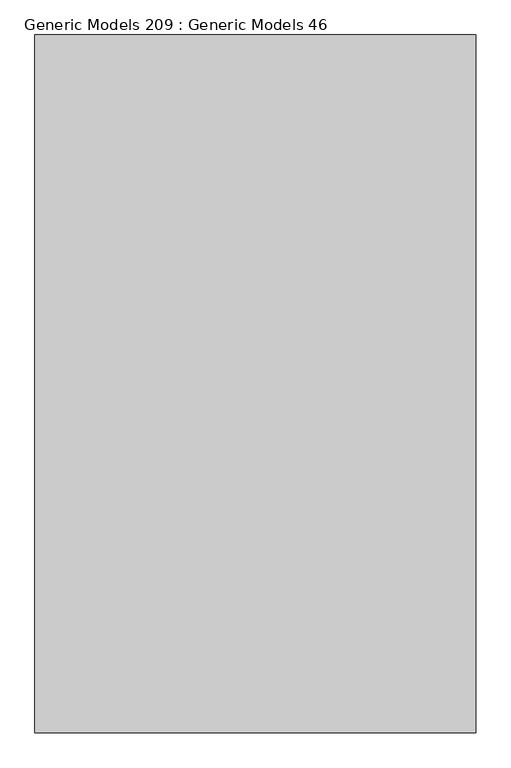
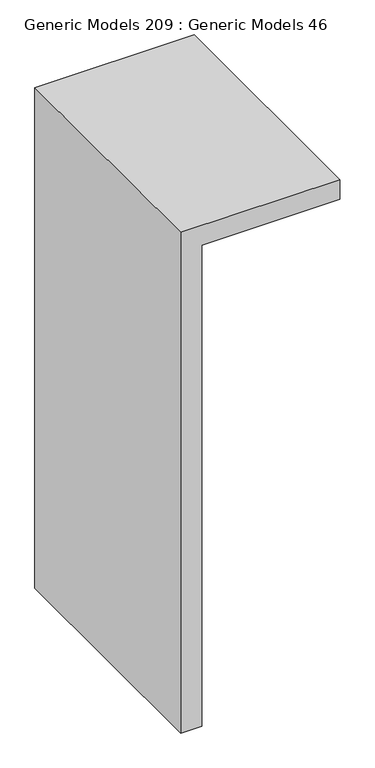
"""IFC4 building model written with IfcOpenShell, lengths in millimetres: proxy geometry, Generic Models 209 : Generic Models 46."""

from ifc_helpers import new_model, si_unit, frame, origin, place, context, project, spatial, polyline, outline, extrude, source, transform, mapped, element, save


def generic_models_209_generic_models_46_237cc0ef(model_context):
    return source(origin(), model_context, "Body", "SweptSolid", [
        extrude(outline(polyline([(634.6026794, 49556.4071108), (634.6026794, 48786.4696108), (-1924.4473206, 48786.4696108), (-1924.4473206, 48888.0696108), (533.0026794, 48888.0696108), (533.0026794, 49556.4071108), (634.6026794, 49556.4071108)])), frame((0.0, 0.0, 0.0), z_axis=(0.0, 1.0, 0.0), x_axis=(0.0, 0.0, 1.0)), (0.0, 0.0, 1.0), 1219.2),
    ])


if __name__ == "__main__":
    model = new_model("IFC4")
    model_context = context("Model", 3, world=origin())
    ifc_project = project(units=[si_unit("LENGTHUNIT", "METRE", prefix="MILLI")], contexts=[model_context])
    site = spatial("IfcSite", under=ifc_project)
    building = spatial("IfcBuilding", under=site)
    placement = place(None, origin())
    generic_models_209_generic_models_46_shape = generic_models_209_generic_models_46_237cc0ef(model_context)
    element("IfcBuildingElementProxy", 1, Name="Generic Models 209 : Generic Models 46", ObjectType="Generic Models 209 : Generic Models 46", at=placement, inside=building, context=model_context, shape_type="MappedRepresentation", body=[
        mapped(generic_models_209_generic_models_46_shape, transform((0.0, 0.0, 0.0), x_axis=(1.0, 0.0, 0.0), y_axis=(0.0, 1.0, 0.0), z_axis=(0.0, 0.0, 1.0))),
    ])
    save(model, "model.ifc")

# Revit data of these elements
# Element 1 (IfcBuildingElementProxy, "Generic Models 209 : Generic Models 46")
#   Materials on its faces: "EXISTING STRUCTURE"
# Materials
#   "EXISTING STRUCTURE": class "Concrete", colour RGB 129 132 118, transparency 0, Description = "Lightweight concrete", Cost = 0
